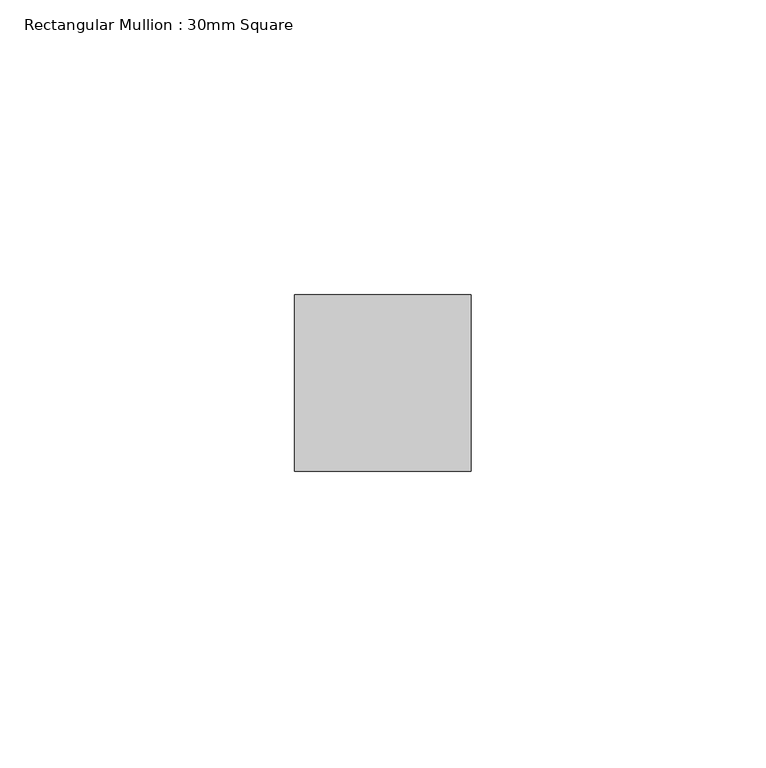
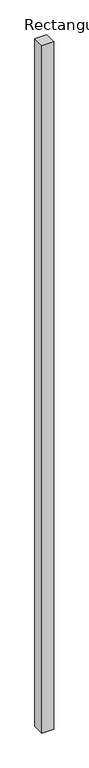
"""IFC4 building model written with IfcOpenShell, lengths in millimetres: member geometry, Rectangular Mullion : 30mm Square."""

from ifc_helpers import new_model, si_unit, frame, origin, place, context, project, spatial, polyline, outline, extrude, source, transform, mapped, element, save


def rectangular_mullion_30mm_square_07de0464(model_context):
    return source(origin(), model_context, "Body", "SweptSolid", [
        extrude(outline(polyline([(15.0, 15.0), (15.0, -15.0), (-15.0, -15.0), (-15.0, 15.0), (15.0, 15.0)])), frame((0.0, 0.0, -1804.8463162), z_axis=(0.0, 0.0, 1.0), x_axis=(1.0, 0.0, 0.0)), (0.0, 0.0, 1.0), 1804.8463162),
    ])


if __name__ == "__main__":
    model = new_model("IFC4")
    model_context = context("Model", 3, world=origin())
    ifc_project = project(units=[si_unit("LENGTHUNIT", "METRE", prefix="MILLI")], contexts=[model_context])
    site = spatial("IfcSite", under=ifc_project)
    building = spatial("IfcBuilding", under=site)
    placement = place(None, origin())
    rectangular_mullion_30mm_square_shape = rectangular_mullion_30mm_square_07de0464(model_context)
    element("IfcMember", 1, ObjectType="Rectangular Mullion : 30mm Square", at=placement, inside=building, context=model_context, shape_type="MappedRepresentation", body=[
        mapped(rectangular_mullion_30mm_square_shape, transform((0.0, 0.0, 0.0), x_axis=(1.0, 0.0, 0.0), y_axis=(0.0, 1.0, 0.0), z_axis=(0.0, 0.0, 1.0))),
    ])
    save(model, "model.ifc")

# Revit data of these elements
# Type "Rectangular Mullion : 30mm Square"
#   built-in parameter 1007304 = 0.0984252 (stored number, unit not read)
#   built-in parameter 1007301 = 0.0492126 (stored number, unit not read)
#   built-in parameter 1007300 = 0.0492126 (stored number, unit not read)
# Element 1 (IfcMember, "Rectangular Mullion : 30mm Square")
#   Materials on its faces: "Aluminum"
# Materials
#   "Aluminum": class "Metal", colour RGB 244 244 244, transparency 0, Description = "Aluminum 6061", Cost = 0
